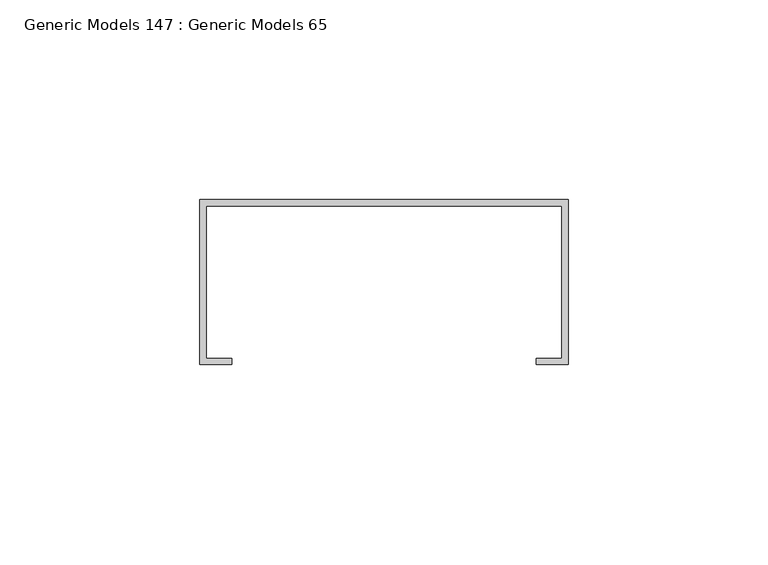
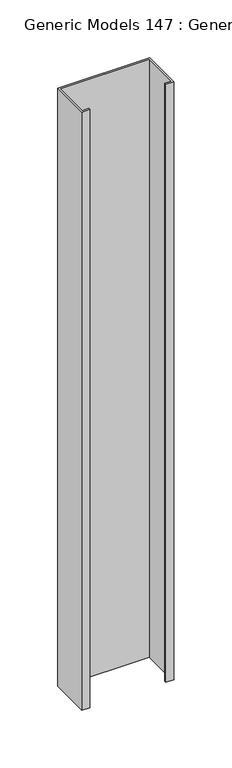
"""IFC4 building model written with IfcOpenShell, lengths in millimetres: proxy geometry, Generic Models 147 : Generic Models 65."""

import ifcopenshell
import ifcopenshell.guid

model = None  # the IFC model being written
_history = None  # IfcOwnerHistory: only IFC2X3 demands one
_inside = {}  # id of a spatial element -> (the spatial element, [elements in it])
_under = {}  # id of a project, library or spatial element -> (it, [spatial elements below it])
_declared = {}  # id of a project -> (the project, [libraries it declares])
_typed = {}  # id of a type object -> (the type object, [elements of that type])
_made_of = {}  # id of a material, layer set ... -> (it, [elements and type objects made of it])


def new_model(schema):
    """Start an empty IFC model of exactly this schema.

    Asked for "IFC4X3", IfcOpenShell would pick the latest addendum, in which some entities
    have other attributes; the version numbers below select the first issue.
    IFC2X3 requires an IfcOwnerHistory on every rooted entity: one is made here for all.
    """
    global model, _history
    if schema == "IFC4X3":
        model = ifcopenshell.file(schema_version=(4, 3, 0, 0))
    else:
        model = ifcopenshell.file(schema=schema)
    _inside.clear()
    _under.clear()
    _declared.clear()
    _typed.clear()
    _made_of.clear()
    _history = None
    if model.schema == "IFC2X3":
        org = make("IfcOrganization", Name="unknown")
        user = make(
            "IfcPersonAndOrganization",
            ThePerson=make("IfcPerson", FamilyName="unknown"),
            TheOrganization=org,
        )
        app = make(
            "IfcApplication",
            ApplicationDeveloper=org,
            Version="unknown",
            ApplicationFullName="unknown",
            ApplicationIdentifier="unknown",
        )
        _history = make(
            "IfcOwnerHistory",
            OwningUser=user,
            OwningApplication=app,
            ChangeAction="ADDED",
            CreationDate=0,
        )
    return model


def make(cls, **values):
    """One entity of the class cls with the attributes given. An attribute that is None is left unset."""
    return model.create_entity(
        cls, **{name: value for name, value in values.items() if value is not None}
    )


def rooted(cls, **values):
    """An entity with a GlobalId (a new one), such as an element, a storey or a relation."""
    return make(cls, GlobalId=ifcopenshell.guid.new(), OwnerHistory=_history, **values)


def si_unit(unit_type, name, prefix=None):
    """IfcSIUnit, for example si_unit("LENGTHUNIT", "METRE", prefix="MILLI")."""
    return make("IfcSIUnit", UnitType=unit_type, Prefix=prefix, Name=name)


def assignment(units):
    """IfcUnitAssignment: the units of a project."""
    return None if units is None else make("IfcUnitAssignment", Units=units)


def point(xyz):
    """IfcCartesianPoint."""
    return None if xyz is None else make("IfcCartesianPoint", Coordinates=xyz)


def direction(xyz):
    """IfcDirection."""
    return None if xyz is None else make("IfcDirection", DirectionRatios=xyz)


def frame(location, z_axis=None, x_axis=None):
    """IfcAxis2Placement3D, a coordinate frame: its origin and axes. An axis left out is left unset."""
    return make(
        "IfcAxis2Placement3D",
        Location=point(location),
        Axis=direction(z_axis),
        RefDirection=direction(x_axis),
    )


def origin():
    """The frame at (0, 0, 0) with its axes left unset."""
    return frame((0.0, 0.0, 0.0))


def place(relative_to, where):
    """IfcLocalPlacement: puts the frame where relative to a parent placement (None: the world)."""
    return make(
        "IfcLocalPlacement", PlacementRelTo=relative_to, RelativePlacement=where
    )


def context(
    kind, dimensions, precision=None, world=None, true_north=None, identifier=None
):
    """IfcGeometricRepresentationContext, for example the 3D "Model" context."""
    return make(
        "IfcGeometricRepresentationContext",
        ContextIdentifier=identifier,
        ContextType=kind,
        CoordinateSpaceDimension=dimensions,
        Precision=precision,
        WorldCoordinateSystem=world,
        TrueNorth=true_north,
    )


def project(units=None, contexts=None):
    """IfcProject with its units and contexts."""
    return rooted(
        "IfcProject",
        Name="project",
        RepresentationContexts=contexts,
        UnitsInContext=assignment(units),
    )


def spatial(cls, under=None, at=None, **own):
    """A site, building, storey or space (cls), placed at a placement, below another one or the project."""
    s = rooted(cls, ObjectPlacement=at, **own)
    if under is not None:
        _under.setdefault(under.id(), (under, []))[1].append(s)
    return s


def polyline(points):
    """IfcPolyline through the points."""
    return make("IfcPolyline", Points=[point(p) for p in points])


def outline(outer, holes=None, kind="AREA"):
    """IfcArbitraryClosedProfileDef: a profile drawn as a closed curve; with holes, ...WithVoids."""
    if holes is None:
        return make("IfcArbitraryClosedProfileDef", ProfileType=kind, OuterCurve=outer)
    return make(
        "IfcArbitraryProfileDefWithVoids",
        ProfileType=kind,
        OuterCurve=outer,
        InnerCurves=holes,
    )


def extrude(swept, where, along, depth):
    """IfcExtrudedAreaSolid: the profile swept, set in the frame where, extruded along a direction by depth."""
    return make(
        "IfcExtrudedAreaSolid",
        SweptArea=swept,
        Position=where,
        ExtrudedDirection=direction(along),
        Depth=depth,
    )


def shape(context_of_items, identifier, shape_type, items):
    """IfcShapeRepresentation: the items that make up one representation, for example the "Body"."""
    return make(
        "IfcShapeRepresentation",
        ContextOfItems=context_of_items,
        RepresentationIdentifier=identifier,
        RepresentationType=shape_type,
        Items=items,
    )


def source(mapping_origin, context_of_items, identifier, shape_type, items):
    """IfcRepresentationMap: a shape defined once, which mapped items show again and again."""
    return make(
        "IfcRepresentationMap",
        MappingOrigin=mapping_origin,
        MappedRepresentation=shape(context_of_items, identifier, shape_type, items),
    )


def transform(
    local_origin,
    x_axis=None,
    y_axis=None,
    z_axis=None,
    scale=None,
    scale2=None,
    scale3=None,
    uniform=True,
):
    """IfcCartesianTransformationOperator3D, or its non-uniform kind. x_axis, y_axis, z_axis: its Axis1, 2, 3."""
    if uniform:
        return make(
            "IfcCartesianTransformationOperator3D",
            Axis1=direction(x_axis),
            Axis2=direction(y_axis),
            LocalOrigin=point(local_origin),
            Scale=scale,
            Axis3=direction(z_axis),
        )
    return make(
        "IfcCartesianTransformationOperator3DnonUniform",
        Axis1=direction(x_axis),
        Axis2=direction(y_axis),
        LocalOrigin=point(local_origin),
        Scale=scale,
        Axis3=direction(z_axis),
        Scale2=scale2,
        Scale3=scale3,
    )


def mapped(mapping_source, mapping_target):
    """IfcMappedItem: shows the shape of a source again, moved by a transform."""
    return make(
        "IfcMappedItem", MappingSource=mapping_source, MappingTarget=mapping_target
    )


def made_of(thing, what):
    """Note that an element or type object is made of a material, layer set ...; save() writes the relation."""
    if what is not None:
        _made_of.setdefault(what.id(), (what, []))[1].append(thing)
    return thing


def element(
    cls,
    number,
    at=None,
    inside=None,
    cuts=None,
    type_object=None,
    material=None,
    context=None,
    identifier="Body",
    shape_type=None,
    held_by="IfcProductDefinitionShape",
    body=None,
    shapes=None,
    **own,
):
    """One element of the class cls, such as IfcWall. Its Tag is "e" and its number.

    at: its placement. inside: the storey or other place that contains it. cuts: it is an
    opening in that element (IfcRelVoidsElement). A single representation is given by context,
    identifier, shape_type and body (its items); several are given by shapes. held_by: the class
    of the entity that holds the representations. save() writes the other relations.
    """
    e = rooted(cls, Tag="e%d" % number, ObjectPlacement=at, **own)
    if body is not None:
        shapes = [shape(context, identifier, shape_type, body)]
    if shapes is not None:
        e.Representation = make(held_by, Representations=shapes)
    if inside is not None:
        _inside.setdefault(inside.id(), (inside, []))[1].append(e)
    if cuts is not None:
        rooted(
            "IfcRelVoidsElement", RelatingBuildingElement=cuts, RelatedOpeningElement=e
        )
    if type_object is not None:
        _typed.setdefault(type_object.id(), (type_object, []))[1].append(e)
    return made_of(e, material)


def aggregate(whole, parts):
    """IfcRelAggregates: a whole, such as a stair, and the parts it consists of."""
    return rooted("IfcRelAggregates", RelatingObject=whole, RelatedObjects=parts)


def save(model, path):
    """Write the relations noted so far, then the file.

    IfcRelAggregates (storeys below a building ...), IfcRelContainedInSpatialStructure (elements
    in a storey), IfcRelDefinesByType, IfcRelAssociatesMaterial and IfcRelDeclares: one each for
    every whole, place, type object, material and project.
    """
    for whole, parts in _under.values():
        aggregate(whole, parts)
    for where, things in _inside.values():
        rooted(
            "IfcRelContainedInSpatialStructure",
            RelatedElements=things,
            RelatingStructure=where,
        )
    for kind, things in _typed.values():
        rooted("IfcRelDefinesByType", RelatedObjects=things, RelatingType=kind)
    for what, things in _made_of.values():
        rooted("IfcRelAssociatesMaterial", RelatedObjects=things, RelatingMaterial=what)
    for by, libraries in _declared.values():
        rooted("IfcRelDeclares", RelatingContext=by, RelatedDefinitions=libraries)
    model.write(path)


def generic_models_147_generic_models_65_32bd72f3(model_context):
    return source(origin(), model_context, "Body", "SweptSolid", [
        extrude(outline(polyline([(50929.4431639, 630.2375), (51021.5181639, 630.2375), (51021.5181639, 588.9625), (51013.5806639, 588.9625), (51013.5806639, 590.55), (51019.9306639, 590.55), (51019.9306639, 628.65), (50931.0306639, 628.65), (50931.0306639, 590.55), (50937.3806639, 590.55), (50937.3806639, 588.9625), (50929.4431639, 588.9625), (50929.4431639, 630.2375)])), frame((0.0, 0.0, -326.1874501), z_axis=(0.0, 0.0, 1.0), x_axis=(1.0, 0.0, 0.0)), (0.0, 0.0, 1.0), 631.6265625),
    ])


if __name__ == "__main__":
    model = new_model("IFC4")
    model_context = context("Model", 3, world=origin())
    ifc_project = project(units=[si_unit("LENGTHUNIT", "METRE", prefix="MILLI")], contexts=[model_context])
    site = spatial("IfcSite", under=ifc_project)
    building = spatial("IfcBuilding", under=site)
    placement = place(None, origin())
    generic_models_147_generic_models_65_shape = generic_models_147_generic_models_65_32bd72f3(model_context)
    element("IfcBuildingElementProxy", 1, Name="Generic Models 147 : Generic Models 65", ObjectType="Generic Models 147 : Generic Models 65", at=placement, inside=building, context=model_context, shape_type="MappedRepresentation", body=[
        mapped(generic_models_147_generic_models_65_shape, transform((0.0, 0.0, 0.0), x_axis=(1.0, 0.0, 0.0), y_axis=(0.0, 1.0, 0.0), z_axis=(0.0, 0.0, 1.0))),
    ])
    save(model, "model.ifc")

# Revit data of these elements
# Element 1 (IfcBuildingElementProxy, "Generic Models 147 : Generic Models 65")
#   Materials on its faces: "METAL STUD (16\" O.C.)"
# Materials
#   "METAL STUD (16\" O.C.)": class "Unassigned", colour RGB 210 209 208, transparency 0, Keynote = "M05121300.02", Cost = 0
